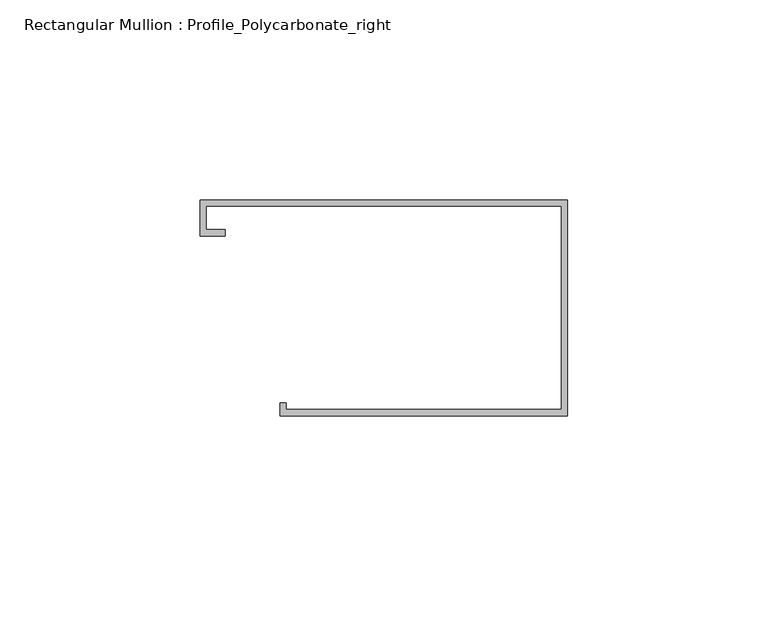
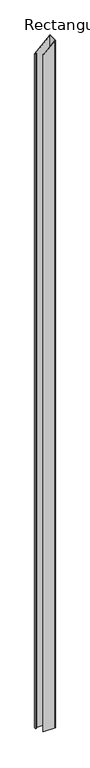
"""IFC4 building model written with IfcOpenShell, lengths in millimetres: member geometry, Rectangular Mullion : Profile_Polycarbonate_right."""

from ifc_helpers import new_model, si_unit, origin, place, context, project, spatial, faceted_brep, source, transform, mapped, element, save


def rectangular_mullion_profile_polycarbonate_right_e3a1531c(model_context):
    return source(origin(), model_context, "Body", "Brep", [
        faceted_brep([(0.0, 28.984575, -4343.796875), (0.0, -25.015825, -4343.796875), (-71.9836, -25.015825, -4343.796875), (-71.9836, -21.840825, -4343.796875), (-70.3961, -21.840825, -4343.796875), (-70.3961, -23.428325, -4343.796875), (-1.5875, -23.428325, -4343.796875), (-1.5875, 27.397075, -4343.796875), (-90.4113, 27.397075, -4343.796875), (-90.4113, 21.580475, -4343.796875), (-85.6488, 21.580475, -4343.796875), (-85.6488, 19.992975, -4343.796875), (-91.9988, 19.992975, -4343.796875), (-91.9988, 28.984575, -4343.796875), (-91.9988, 28.984575, -88.2453421), (0.0, 28.984575, 0.0), (-91.9988, 19.992975, -88.2453421), (-85.6488, 19.992975, -82.1544157), (-85.6488, 21.580475, -82.1544157), (-90.4113, 21.580475, -86.7226105), (-90.4113, 27.397075, -86.7226105), (-1.5875, 27.397075, -1.5227316), (-1.5875, -23.428325, -1.5227316), (-70.3961, -23.428325, -67.5240104), (-70.3961, -21.840825, -67.5240104), (-71.9836, -21.840825, -69.046742), (-71.9836, -25.015825, -69.046742), (0.0, -25.015825, 0.0)], [[[0, 1, 2, 3, 4, 5, 6, 7, 8, 9, 10, 11, 12, 13]], [[14, 15, 0, 13]], [[16, 14, 13, 12]], [[17, 16, 12, 11]], [[18, 17, 11, 10]], [[19, 18, 10, 9]], [[20, 19, 9, 8]], [[21, 20, 8, 7]], [[22, 21, 7, 6]], [[23, 22, 6, 5]], [[24, 23, 5, 4]], [[25, 24, 4, 3]], [[26, 25, 3, 2]], [[27, 26, 2, 1]], [[15, 27, 1, 0]], [[15, 14, 16, 17, 18, 19, 20, 21, 22, 23, 24, 25, 26, 27]]]),
    ])


if __name__ == "__main__":
    model = new_model("IFC4")
    model_context = context("Model", 3, world=origin())
    ifc_project = project(units=[si_unit("LENGTHUNIT", "METRE", prefix="MILLI")], contexts=[model_context])
    site = spatial("IfcSite", under=ifc_project)
    building = spatial("IfcBuilding", under=site)
    placement = place(None, origin())
    rectangular_mullion_profile_polycarbonate_right_shape = rectangular_mullion_profile_polycarbonate_right_e3a1531c(model_context)
    element("IfcMember", 1, ObjectType="Rectangular Mullion : Profile_Polycarbonate_right", at=placement, inside=building, context=model_context, shape_type="MappedRepresentation", body=[
        mapped(rectangular_mullion_profile_polycarbonate_right_shape, transform((0.0, 0.0, 0.0), x_axis=(1.0, 0.0, 0.0), y_axis=(0.0, 1.0, 0.0), z_axis=(0.0, 0.0, 1.0))),
    ])
    save(model, "model.ifc")

# Revit data of these elements
# Type "Rectangular Mullion : Profile_Polycarbonate_right"
#   built-in parameter 1007322 = 0.177167 (stored number, unit not read)
#   built-in parameter 1007321 = 0 (stored number, unit not read)
#   built-in parameter 1007320 = 0.00520833 (stored number, unit not read)
